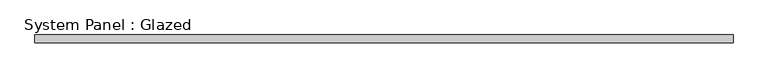
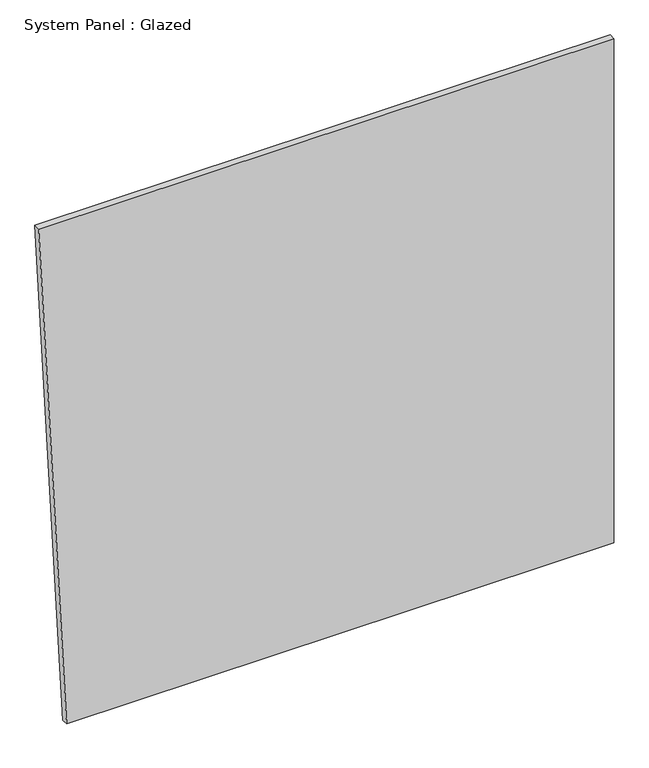
"""IFC4 building model written with IfcOpenShell, lengths in millimetres: plate geometry, System Panel : Glazed."""

import ifcopenshell
import ifcopenshell.guid

model = None  # the IFC model being written
_history = None  # IfcOwnerHistory: only IFC2X3 demands one
_inside = {}  # id of a spatial element -> (the spatial element, [elements in it])
_under = {}  # id of a project, library or spatial element -> (it, [spatial elements below it])
_declared = {}  # id of a project -> (the project, [libraries it declares])
_typed = {}  # id of a type object -> (the type object, [elements of that type])
_made_of = {}  # id of a material, layer set ... -> (it, [elements and type objects made of it])


def new_model(schema):
    """Start an empty IFC model of exactly this schema.

    Asked for "IFC4X3", IfcOpenShell would pick the latest addendum, in which some entities
    have other attributes; the version numbers below select the first issue.
    IFC2X3 requires an IfcOwnerHistory on every rooted entity: one is made here for all.
    """
    global model, _history
    if schema == "IFC4X3":
        model = ifcopenshell.file(schema_version=(4, 3, 0, 0))
    else:
        model = ifcopenshell.file(schema=schema)
    _inside.clear()
    _under.clear()
    _declared.clear()
    _typed.clear()
    _made_of.clear()
    _history = None
    if model.schema == "IFC2X3":
        org = make("IfcOrganization", Name="unknown")
        user = make(
            "IfcPersonAndOrganization",
            ThePerson=make("IfcPerson", FamilyName="unknown"),
            TheOrganization=org,
        )
        app = make(
            "IfcApplication",
            ApplicationDeveloper=org,
            Version="unknown",
            ApplicationFullName="unknown",
            ApplicationIdentifier="unknown",
        )
        _history = make(
            "IfcOwnerHistory",
            OwningUser=user,
            OwningApplication=app,
            ChangeAction="ADDED",
            CreationDate=0,
        )
    return model


def make(cls, **values):
    """One entity of the class cls with the attributes given. An attribute that is None is left unset."""
    return model.create_entity(
        cls, **{name: value for name, value in values.items() if value is not None}
    )


def rooted(cls, **values):
    """An entity with a GlobalId (a new one), such as an element, a storey or a relation."""
    return make(cls, GlobalId=ifcopenshell.guid.new(), OwnerHistory=_history, **values)


def si_unit(unit_type, name, prefix=None):
    """IfcSIUnit, for example si_unit("LENGTHUNIT", "METRE", prefix="MILLI")."""
    return make("IfcSIUnit", UnitType=unit_type, Prefix=prefix, Name=name)


def assignment(units):
    """IfcUnitAssignment: the units of a project."""
    return None if units is None else make("IfcUnitAssignment", Units=units)


def point(xyz):
    """IfcCartesianPoint."""
    return None if xyz is None else make("IfcCartesianPoint", Coordinates=xyz)


def direction(xyz):
    """IfcDirection."""
    return None if xyz is None else make("IfcDirection", DirectionRatios=xyz)


def frame(location, z_axis=None, x_axis=None):
    """IfcAxis2Placement3D, a coordinate frame: its origin and axes. An axis left out is left unset."""
    return make(
        "IfcAxis2Placement3D",
        Location=point(location),
        Axis=direction(z_axis),
        RefDirection=direction(x_axis),
    )


def origin():
    """The frame at (0, 0, 0) with its axes left unset."""
    return frame((0.0, 0.0, 0.0))


def place(relative_to, where):
    """IfcLocalPlacement: puts the frame where relative to a parent placement (None: the world)."""
    return make(
        "IfcLocalPlacement", PlacementRelTo=relative_to, RelativePlacement=where
    )


def context(
    kind, dimensions, precision=None, world=None, true_north=None, identifier=None
):
    """IfcGeometricRepresentationContext, for example the 3D "Model" context."""
    return make(
        "IfcGeometricRepresentationContext",
        ContextIdentifier=identifier,
        ContextType=kind,
        CoordinateSpaceDimension=dimensions,
        Precision=precision,
        WorldCoordinateSystem=world,
        TrueNorth=true_north,
    )


def project(units=None, contexts=None):
    """IfcProject with its units and contexts."""
    return rooted(
        "IfcProject",
        Name="project",
        RepresentationContexts=contexts,
        UnitsInContext=assignment(units),
    )


def spatial(cls, under=None, at=None, **own):
    """A site, building, storey or space (cls), placed at a placement, below another one or the project."""
    s = rooted(cls, ObjectPlacement=at, **own)
    if under is not None:
        _under.setdefault(under.id(), (under, []))[1].append(s)
    return s


def polyline(points):
    """IfcPolyline through the points."""
    return make("IfcPolyline", Points=[point(p) for p in points])


def outline(outer, holes=None, kind="AREA"):
    """IfcArbitraryClosedProfileDef: a profile drawn as a closed curve; with holes, ...WithVoids."""
    if holes is None:
        return make("IfcArbitraryClosedProfileDef", ProfileType=kind, OuterCurve=outer)
    return make(
        "IfcArbitraryProfileDefWithVoids",
        ProfileType=kind,
        OuterCurve=outer,
        InnerCurves=holes,
    )


def extrude(swept, where, along, depth):
    """IfcExtrudedAreaSolid: the profile swept, set in the frame where, extruded along a direction by depth."""
    return make(
        "IfcExtrudedAreaSolid",
        SweptArea=swept,
        Position=where,
        ExtrudedDirection=direction(along),
        Depth=depth,
    )


def shape(context_of_items, identifier, shape_type, items):
    """IfcShapeRepresentation: the items that make up one representation, for example the "Body"."""
    return make(
        "IfcShapeRepresentation",
        ContextOfItems=context_of_items,
        RepresentationIdentifier=identifier,
        RepresentationType=shape_type,
        Items=items,
    )


def source(mapping_origin, context_of_items, identifier, shape_type, items):
    """IfcRepresentationMap: a shape defined once, which mapped items show again and again."""
    return make(
        "IfcRepresentationMap",
        MappingOrigin=mapping_origin,
        MappedRepresentation=shape(context_of_items, identifier, shape_type, items),
    )


def transform(
    local_origin,
    x_axis=None,
    y_axis=None,
    z_axis=None,
    scale=None,
    scale2=None,
    scale3=None,
    uniform=True,
):
    """IfcCartesianTransformationOperator3D, or its non-uniform kind. x_axis, y_axis, z_axis: its Axis1, 2, 3."""
    if uniform:
        return make(
            "IfcCartesianTransformationOperator3D",
            Axis1=direction(x_axis),
            Axis2=direction(y_axis),
            LocalOrigin=point(local_origin),
            Scale=scale,
            Axis3=direction(z_axis),
        )
    return make(
        "IfcCartesianTransformationOperator3DnonUniform",
        Axis1=direction(x_axis),
        Axis2=direction(y_axis),
        LocalOrigin=point(local_origin),
        Scale=scale,
        Axis3=direction(z_axis),
        Scale2=scale2,
        Scale3=scale3,
    )


def mapped(mapping_source, mapping_target):
    """IfcMappedItem: shows the shape of a source again, moved by a transform."""
    return make(
        "IfcMappedItem", MappingSource=mapping_source, MappingTarget=mapping_target
    )


def made_of(thing, what):
    """Note that an element or type object is made of a material, layer set ...; save() writes the relation."""
    if what is not None:
        _made_of.setdefault(what.id(), (what, []))[1].append(thing)
    return thing


def element(
    cls,
    number,
    at=None,
    inside=None,
    cuts=None,
    type_object=None,
    material=None,
    context=None,
    identifier="Body",
    shape_type=None,
    held_by="IfcProductDefinitionShape",
    body=None,
    shapes=None,
    **own,
):
    """One element of the class cls, such as IfcWall. Its Tag is "e" and its number.

    at: its placement. inside: the storey or other place that contains it. cuts: it is an
    opening in that element (IfcRelVoidsElement). A single representation is given by context,
    identifier, shape_type and body (its items); several are given by shapes. held_by: the class
    of the entity that holds the representations. save() writes the other relations.
    """
    e = rooted(cls, Tag="e%d" % number, ObjectPlacement=at, **own)
    if body is not None:
        shapes = [shape(context, identifier, shape_type, body)]
    if shapes is not None:
        e.Representation = make(held_by, Representations=shapes)
    if inside is not None:
        _inside.setdefault(inside.id(), (inside, []))[1].append(e)
    if cuts is not None:
        rooted(
            "IfcRelVoidsElement", RelatingBuildingElement=cuts, RelatedOpeningElement=e
        )
    if type_object is not None:
        _typed.setdefault(type_object.id(), (type_object, []))[1].append(e)
    return made_of(e, material)


def aggregate(whole, parts):
    """IfcRelAggregates: a whole, such as a stair, and the parts it consists of."""
    return rooted("IfcRelAggregates", RelatingObject=whole, RelatedObjects=parts)


def save(model, path):
    """Write the relations noted so far, then the file.

    IfcRelAggregates (storeys below a building ...), IfcRelContainedInSpatialStructure (elements
    in a storey), IfcRelDefinesByType, IfcRelAssociatesMaterial and IfcRelDeclares: one each for
    every whole, place, type object, material and project.
    """
    for whole, parts in _under.values():
        aggregate(whole, parts)
    for where, things in _inside.values():
        rooted(
            "IfcRelContainedInSpatialStructure",
            RelatedElements=things,
            RelatingStructure=where,
        )
    for kind, things in _typed.values():
        rooted("IfcRelDefinesByType", RelatedObjects=things, RelatingType=kind)
    for what, things in _made_of.values():
        rooted("IfcRelAssociatesMaterial", RelatedObjects=things, RelatingMaterial=what)
    for by, libraries in _declared.values():
        rooted("IfcRelDeclares", RelatingContext=by, RelatedDefinitions=libraries)
    model.write(path)


def system_panel_glazed_282f07fc(model_context):
    return source(origin(), model_context, "Body", "SweptSolid", [
        extrude(outline(polyline([(0.0, -1017.0034845), (0.0, 1126.1853377), (2086.1728929, 1126.1853377), (2086.1728929, -1126.1853377), (0.0, -1017.0034845)])), frame((0.0, -44.45, 0.0), z_axis=(0.0, 1.0, 0.0), x_axis=(0.0, 0.0, 1.0)), (0.0, 0.0, 1.0), 25.4),
    ])


if __name__ == "__main__":
    model = new_model("IFC4")
    model_context = context("Model", 3, world=origin())
    ifc_project = project(units=[si_unit("LENGTHUNIT", "METRE", prefix="MILLI")], contexts=[model_context])
    site = spatial("IfcSite", under=ifc_project)
    building = spatial("IfcBuilding", under=site)
    placement = place(None, origin())
    system_panel_glazed_shape = system_panel_glazed_282f07fc(model_context)
    element("IfcPlate", 1, ObjectType="System Panel : Glazed", at=placement, inside=building, context=model_context, shape_type="MappedRepresentation", body=[
        mapped(system_panel_glazed_shape, transform((0.0, 0.0, 0.0), x_axis=(1.0, 0.0, 0.0), y_axis=(0.0, 1.0, 0.0), z_axis=(0.0, 0.0, 1.0))),
    ])
    save(model, "model.ifc")

# Revit data of these elements
# Type "System Panel : Glazed"
#   Construction Type Id = "GSP4R"
#   Analytic Construction = "1/8 in Pilkington single glazing"
#   Visual Light Transmittance = 0.9
#   Solar Heat Gain Coefficient = 0.86
#   Heat Transfer Coefficient (U) = 1.18115 BTU/(h·ft²·°F)
#   Define Thermal Properties by = 1
# Element 1 (IfcPlate, "System Panel : Glazed")
#   Materials on its faces: "Glass"
# Materials
#   "Glass": class "Glass", colour RGB 0 128 192, transparency 0.75, Description = "Soda Lime Glass", Cost = 0
